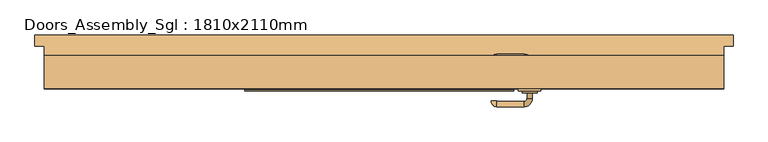
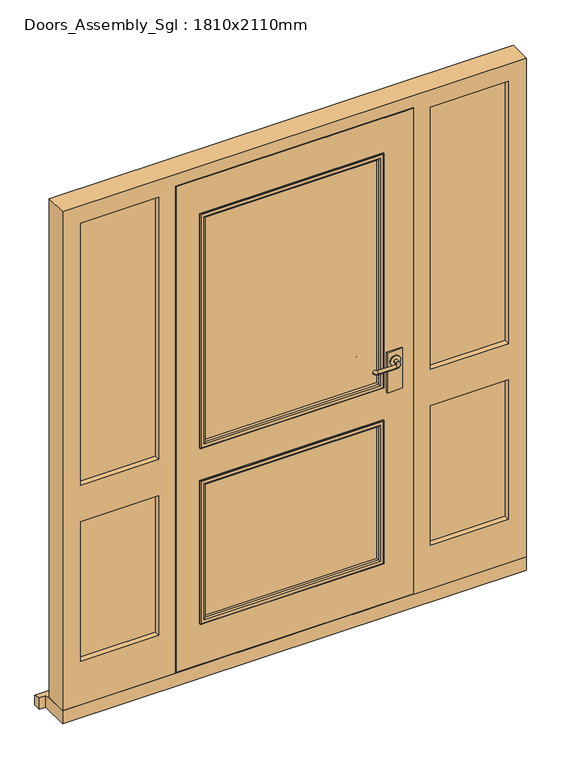
"""IFC4 building model written with IfcOpenShell, lengths in millimetres: door geometry, Doors_Assembly_Sgl : 1810x2110mm."""

from ifc_helpers import new_model, si_unit, point, frame, frame_2d, origin, place, context, project, spatial, polyline, circle_curve, ellipse_curve, trimmed, segment, composite_curve, outline, extrude, faceted_brep, source, transform, mapped, element, save
from ifc_brep_helpers import plane_surface, cylinder_surface, revolved_surface, advanced_brep


def doors_assembly_sgl_1810x2110mm_9edc52a6(model_context):
    return source(origin(), model_context, "Body", "SolidModel", [
        extrude(outline(composite_curve([segment(trimmed(circle_curve(frame_2d((1050.0, 680.0)), 20.0), [point((1050.0, 700.0))], [point((1050.0, 660.0))], False, "CARTESIAN"), True, "CONTINUOUS"), segment(trimmed(circle_curve(frame_2d((1050.0, 680.0)), 20.0), [point((1050.0, 660.0))], [point((1050.0, 700.0))], False, "CARTESIAN"), True, "CONTINUOUS")], self_intersect=False)), frame((0.0, 41.6570105, 0.0), z_axis=(0.0, 1.0, 0.0), x_axis=(0.0, 0.0, 1.0)), (0.0, 0.0, 1.0), 4.5929895),
        advanced_brep(
        [(673.0, 41.6570105, 1050.0), (687.0, 41.6570105, 1050.0), (673.0, 26.25, 1050.0), (687.0, 26.25, 1050.0), (665.0, 4.25, 1050.0), (665.0, 18.25, 1050.0), (593.0, 18.25, 1050.0), (593.0, 4.25, 1050.0), (592.0, 19.25, 1050.0), (578.0, 19.25, 1050.0)],
        [
            (0, 1, circle_curve(frame((680.0, 41.6570105, 1050.0), z_axis=(0.0, 1.0, 0.0), x_axis=(1.0, 0.0, 0.0)), 7.0)),
            (1, 0, circle_curve(frame((680.0, 41.6570105, 1050.0), z_axis=(0.0, 1.0, 0.0), x_axis=(1.0, 0.0, 0.0)), 7.0)),
            (0, 2),
            (2, 3, circle_curve(frame((680.0, 26.25, 1050.0), z_axis=(0.0, 1.0, 0.0), x_axis=(1.0, 0.0, 0.0)), 7.0)),
            (3, 1),
            (3, 2, circle_curve(frame((680.0, 26.25, 1050.0), z_axis=(0.0, 1.0, 0.0), x_axis=(1.0, 0.0, 0.0)), 7.0)),
            (4, 3, circle_curve(frame((665.0, 26.25, 1050.0), z_axis=(0.0, 0.0, 1.0), x_axis=(1.0, 0.0, 0.0)), 22.0)),
            (2, 5, circle_curve(frame((665.0, 26.25, 1050.0), z_axis=(0.0, 0.0, -1.0), x_axis=(1.0, 0.0, 0.0)), 8.0)),
            (5, 4, circle_curve(frame((665.0, 11.25, 1050.0), z_axis=(1.0, 0.0, 0.0), x_axis=(0.0, -1.0, 0.0)), 7.0)),
            (4, 5, circle_curve(frame((665.0, 11.25, 1050.0), z_axis=(1.0, 0.0, 0.0), x_axis=(0.0, -1.0, 0.0)), 7.0)),
            (5, 6),
            (6, 7, circle_curve(frame((593.0, 11.25, 1050.0), z_axis=(1.0, 0.0, 0.0), x_axis=(0.0, -1.0, 0.0)), 7.0)),
            (7, 4),
            (7, 6, circle_curve(frame((593.0, 11.25, 1050.0), z_axis=(1.0, 0.0, 0.0), x_axis=(0.0, -1.0, 0.0)), 7.0)),
            (8, 9, circle_curve(frame((585.0, 19.25, 1050.0), z_axis=(0.0, 1.0, 0.0), x_axis=(-1.0, 0.0, 0.0)), 7.0)),
            (9, 8, circle_curve(frame((585.0, 19.25, 1050.0), z_axis=(0.0, 1.0, 0.0), x_axis=(-1.0, 0.0, 0.0)), 7.0)),
            (9, 7, circle_curve(frame((593.0, 19.25, 1050.0), z_axis=(0.0, 0.0, 1.0), x_axis=(0.0, -1.0, 0.0)), 15.0)),
            (6, 8, circle_curve(frame((593.0, 19.25, 1050.0), z_axis=(0.0, 0.0, -1.0), x_axis=(0.0, -1.0, 0.0)), 1.0)),
        ],
        [
            plane_surface(frame((680.0, 41.6570105, 1050.0), z_axis=(0.0, 1.0, 0.0), x_axis=(0.0, 0.0, 1.0))),
            cylinder_surface(frame((680.0, 41.6570105, 1050.0), z_axis=(0.0, 1.0, 0.0), x_axis=(1.0, 0.0, 0.0)), 7.0),
            revolved_surface(trimmed(ellipse_curve(frame((680.0, 26.25, 1050.0), z_axis=(0.0, 1.0, 0.0), x_axis=(1.0, 0.0, 0.0)), 7.0, 7.0), [point((673.0, 26.25, 1050.0))], [point((687.0, 26.25, 1050.0))], True, "CARTESIAN"), (665.0, 26.25, 1050.0), (0.0, 0.0, -1.0)),
            revolved_surface(trimmed(ellipse_curve(frame((680.0, 26.25, 1050.0), z_axis=(0.0, 1.0, 0.0), x_axis=(1.0, 0.0, 0.0)), 7.0, 7.0), [point((687.0, 26.25, 1050.0))], [point((673.0, 26.25, 1050.0))], True, "CARTESIAN"), (665.0, 26.25, 1050.0), (0.0, 0.0, -1.0)),
            cylinder_surface(frame((665.0, 11.25, 1050.0), z_axis=(1.0, 0.0, 0.0), x_axis=(0.0, -1.0, 0.0)), 7.0),
            plane_surface(frame((585.0, 19.25, 1050.0), z_axis=(0.0, 1.0, 0.0), x_axis=(0.0, 0.0, 1.0))),
            revolved_surface(trimmed(ellipse_curve(frame((593.0, 11.25, 1050.0), z_axis=(1.0, 0.0, 0.0), x_axis=(0.0, -1.0, 0.0)), 7.0, 7.0), [point((593.0, 18.25, 1050.0))], [point((593.0, 4.25, 1050.0))], True, "CARTESIAN"), (593.0, 19.25, 1050.0), (0.0, 0.0, -1.0)),
            revolved_surface(trimmed(ellipse_curve(frame((593.0, 11.25, 1050.0), z_axis=(1.0, 0.0, 0.0), x_axis=(0.0, -1.0, 0.0)), 7.0, 7.0), [point((593.0, 4.25, 1050.0))], [point((593.0, 18.25, 1050.0))], True, "CARTESIAN"), (593.0, 19.25, 1050.0), (0.0, 0.0, -1.0)),
        ],
        [
            (0, [[1, 2]]),
            (1, [[-1, 3, 4, 5]]),
            (1, [[-2, -5, 6, -3]]),
            (2, [[7, -4, 8, 9]]),
            (3, [[-8, -6, -7, 10]]),
            (4, [[-9, 11, 12, 13]]),
            (4, [[-10, -13, 14, -11]]),
            (5, [[15, 16]]),
            (6, [[17, -12, 18, -16]]),
            (7, [[-18, -14, -17, -15]]),
        ],
    ),
        extrude(outline(polyline([(650.0, 52.25), (710.0, 52.25), (710.0, 46.25), (650.0, 46.25), (650.0, 52.25)])), frame((0.0, 0.0, 925.0), z_axis=(0.0, 0.0, 1.0), x_axis=(1.0, 0.0, 0.0)), (0.0, 0.0, 1.0), 165.0),
        extrude(outline(composite_curve([segment(trimmed(circle_curve(frame_2d((1050.0, 680.0)), 20.0), [point((1050.0, 700.0))], [point((1050.0, 660.0))], False, "CARTESIAN"), True, "CONTINUOUS"), segment(trimmed(circle_curve(frame_2d((1050.0, 680.0)), 20.0), [point((1050.0, 660.0))], [point((1050.0, 700.0))], False, "CARTESIAN"), True, "CONTINUOUS")], self_intersect=False)), frame((0.0, 102.25, 0.0), z_axis=(0.0, 1.0, 0.0), x_axis=(0.0, 0.0, 1.0)), (0.0, 0.0, 1.0), 4.5929895),
        advanced_brep(
        [(673.0, 106.8429895, 1050.0), (687.0, 106.8429895, 1050.0), (687.0, 122.25, 1050.0), (673.0, 122.25, 1050.0), (665.0, 144.25, 1050.0), (665.0, 130.25, 1050.0), (593.0, 144.25, 1050.0), (593.0, 130.25, 1050.0), (592.0, 129.25, 1050.0), (578.0, 129.25, 1050.0)],
        [
            (0, 1, circle_curve(frame((680.0, 106.8429895, 1050.0), z_axis=(0.0, -1.0, 0.0), x_axis=(1.0, 0.0, 0.0)), 7.0)),
            (1, 0, circle_curve(frame((680.0, 106.8429895, 1050.0), z_axis=(0.0, -1.0, 0.0), x_axis=(1.0, 0.0, 0.0)), 7.0)),
            (1, 2),
            (2, 3, circle_curve(frame((680.0, 122.25, 1050.0), z_axis=(0.0, -1.0, 0.0), x_axis=(1.0, 0.0, 0.0)), 7.0)),
            (3, 0),
            (3, 2, circle_curve(frame((680.0, 122.25, 1050.0), z_axis=(0.0, -1.0, 0.0), x_axis=(1.0, 0.0, 0.0)), 7.0)),
            (4, 5, circle_curve(frame((665.0, 137.25, 1050.0), z_axis=(1.0, 0.0, 0.0), x_axis=(0.0, 1.0, 0.0)), 7.0)),
            (5, 3, circle_curve(frame((665.0, 122.25, 1050.0), z_axis=(0.0, 0.0, -1.0), x_axis=(1.0, 0.0, 0.0)), 8.0)),
            (2, 4, circle_curve(frame((665.0, 122.25, 1050.0), z_axis=(0.0, 0.0, 1.0), x_axis=(1.0, 0.0, 0.0)), 22.0)),
            (5, 4, circle_curve(frame((665.0, 137.25, 1050.0), z_axis=(1.0, 0.0, 0.0), x_axis=(0.0, 1.0, 0.0)), 7.0)),
            (4, 6),
            (6, 7, circle_curve(frame((593.0, 137.25, 1050.0), z_axis=(1.0, 0.0, 0.0), x_axis=(0.0, 1.0, 0.0)), 7.0)),
            (7, 5),
            (7, 6, circle_curve(frame((593.0, 137.25, 1050.0), z_axis=(1.0, 0.0, 0.0), x_axis=(0.0, 1.0, 0.0)), 7.0)),
            (8, 9, circle_curve(frame((585.0, 129.25, 1050.0), z_axis=(0.0, -1.0, 0.0), x_axis=(-1.0, 0.0, 0.0)), 7.0)),
            (9, 8, circle_curve(frame((585.0, 129.25, 1050.0), z_axis=(0.0, -1.0, 0.0), x_axis=(-1.0, 0.0, 0.0)), 7.0)),
            (8, 7, circle_curve(frame((593.0, 129.25, 1050.0), z_axis=(0.0, 0.0, -1.0), x_axis=(0.0, 1.0, 0.0)), 1.0)),
            (6, 9, circle_curve(frame((593.0, 129.25, 1050.0), z_axis=(0.0, 0.0, 1.0), x_axis=(0.0, 1.0, 0.0)), 15.0)),
        ],
        [
            plane_surface(frame((680.0, 106.8429895, 1050.0), z_axis=(0.0, -1.0, 0.0), x_axis=(0.0, 0.0, 1.0))),
            cylinder_surface(frame((680.0, 106.8429895, 1050.0), z_axis=(0.0, -1.0, 0.0), x_axis=(1.0, 0.0, 0.0)), 7.0),
            revolved_surface(trimmed(ellipse_curve(frame((680.0, 122.25, 1050.0), z_axis=(0.0, 1.0, 0.0), x_axis=(1.0, 0.0, 0.0)), 7.0, 7.0), [point((673.0, 122.25, 1050.0))], [point((687.0, 122.25, 1050.0))], True, "CARTESIAN"), (665.0, 122.25, 1050.0), (0.0, 0.0, -1.0)),
            revolved_surface(trimmed(ellipse_curve(frame((680.0, 122.25, 1050.0), z_axis=(0.0, 1.0, 0.0), x_axis=(1.0, 0.0, 0.0)), 7.0, 7.0), [point((687.0, 122.25, 1050.0))], [point((673.0, 122.25, 1050.0))], True, "CARTESIAN"), (665.0, 122.25, 1050.0), (0.0, 0.0, -1.0)),
            cylinder_surface(frame((665.0, 137.25, 1050.0), z_axis=(1.0, 0.0, 0.0), x_axis=(0.0, 1.0, 0.0)), 7.0),
            plane_surface(frame((585.0, 129.25, 1050.0), z_axis=(0.0, -1.0, 0.0), x_axis=(0.0, 0.0, 1.0))),
            revolved_surface(trimmed(ellipse_curve(frame((593.0, 137.25, 1050.0), z_axis=(-1.0, 0.0, 0.0), x_axis=(0.0, 1.0, 0.0)), 7.0, 7.0), [point((593.0, 130.25, 1050.0))], [point((593.0, 144.25, 1050.0))], True, "CARTESIAN"), (593.0, 129.25, 1050.0), (0.0, 0.0, -1.0)),
            revolved_surface(trimmed(ellipse_curve(frame((593.0, 137.25, 1050.0), z_axis=(-1.0, 0.0, 0.0), x_axis=(0.0, 1.0, 0.0)), 7.0, 7.0), [point((593.0, 144.25, 1050.0))], [point((593.0, 130.25, 1050.0))], True, "CARTESIAN"), (593.0, 129.25, 1050.0), (0.0, 0.0, -1.0)),
        ],
        [
            (0, [[1, 2]]),
            (1, [[3, 4, 5, -2]]),
            (1, [[-5, 6, -3, -1]]),
            (2, [[7, 8, -4, 9]]),
            (3, [[10, -9, -6, -8]]),
            (4, [[11, 12, 13, -7]]),
            (4, [[-13, 14, -11, -10]]),
            (5, [[15, 16]]),
            (6, [[-15, 17, -12, 18]]),
            (7, [[-16, -18, -14, -17]]),
        ],
    ),
        extrude(outline(polyline([(650.0, 96.25), (650.0, 102.25), (710.0, 102.25), (710.0, 96.25), (650.0, 96.25)])), frame((0.0, 0.0, 925.0), z_axis=(0.0, 0.0, 1.0), x_axis=(1.0, 0.0, 0.0)), (0.0, 0.0, 1.0), 165.0),
        extrude(outline(polyline([(1148.5, 75.25), (800.0, 75.25), (800.0, 99.25), (1148.5, 99.25), (1148.5, 75.25)])), frame((0.0, 0.0, 218.5), z_axis=(0.0, 0.0, 1.0), x_axis=(1.0, 0.0, 0.0)), (0.0, 0.0, 1.0), 605.0),
        extrude(outline(polyline([(1148.5, 75.25), (800.0, 75.25), (800.0, 99.25), (1148.5, 99.25), (1148.5, 75.25)])), frame((0.0, 0.0, 943.5), z_axis=(0.0, 0.0, 1.0), x_axis=(1.0, 0.0, 0.0)), (0.0, 0.0, 1.0), 1118.0),
        extrude(outline(polyline([(-216.0, 75.25), (-564.5, 75.25), (-564.5, 99.25), (-216.0, 99.25), (-216.0, 75.25)])), frame((0.0, 0.0, 943.5), z_axis=(0.0, 0.0, 1.0), x_axis=(1.0, 0.0, 0.0)), (0.0, 0.0, 1.0), 1118.0),
        extrude(outline(polyline([(-216.0, 75.25), (-564.5, 75.25), (-564.5, 99.25), (-216.0, 99.25), (-216.0, 75.25)])), frame((0.0, 0.0, 218.5), z_axis=(0.0, 0.0, 1.0), x_axis=(1.0, 0.0, 0.0)), (0.0, 0.0, 1.0), 605.0),
        faceted_brep([(1197.0, 141.25, 54.5), (1197.0, 52.25, 54.5), (758.0, 52.25, 54.5), (758.0, 99.25, 54.5), (736.0, 99.25, 54.5), (736.0, 141.25, 54.5), (1197.0, 141.25, 2110.0), (1197.0, 52.25, 2110.0), (-613.0, 52.25, 2110.0), (-613.0, 52.25, 54.5), (-174.0, 52.25, 54.5), (-174.0, 52.25, 2061.5), (758.0, 52.25, 2061.5), (1126.5, 52.25, 958.5), (822.0, 52.25, 958.5), (822.0, 52.25, 2039.5), (1126.5, 52.25, 2039.5), (822.0, 52.25, 808.5), (1126.5, 52.25, 808.5), (1126.5, 52.25, 233.5), (822.0, 52.25, 233.5), (-238.0, 52.25, 808.5), (-238.0, 52.25, 233.5), (-542.5, 52.25, 233.5), (-542.5, 52.25, 808.5), (-542.5, 52.25, 2039.5), (-238.0, 52.25, 2039.5), (-238.0, 52.25, 958.5), (-542.5, 52.25, 958.5), (758.0, 99.25, 2061.5), (-174.0, 99.25, 54.5), (-152.0, 99.25, 54.5), (-152.0, 99.25, 2039.5), (736.0, 99.25, 2039.5), (-174.0, 99.25, 2061.5), (1148.5, 99.25, 218.5), (1148.5, 99.25, 823.5), (800.0, 99.25, 823.5), (800.0, 99.25, 218.5), (1126.5, 99.25, 808.5), (1126.5, 99.25, 233.5), (822.0, 99.25, 233.5), (822.0, 99.25, 808.5), (-564.5, 99.25, 823.5), (-564.5, 99.25, 218.5), (-216.0, 99.25, 218.5), (-216.0, 99.25, 823.5), (-238.0, 99.25, 808.5), (-238.0, 99.25, 233.5), (-542.5, 99.25, 233.5), (-542.5, 99.25, 808.5), (-216.0, 99.25, 2061.5), (-564.5, 99.25, 2061.5), (-564.5, 99.25, 943.5), (-216.0, 99.25, 943.5), (-542.5, 99.25, 2039.5), (-238.0, 99.25, 2039.5), (-238.0, 99.25, 958.5), (-542.5, 99.25, 958.5), (1148.5, 99.25, 2061.5), (800.0, 99.25, 2061.5), (800.0, 99.25, 943.5), (1148.5, 99.25, 943.5), (822.0, 99.25, 2039.5), (1126.5, 99.25, 2039.5), (1126.5, 99.25, 958.5), (822.0, 99.25, 958.5), (736.0, 141.25, 2039.5), (-613.0, 141.25, 54.5), (-613.0, 141.25, 2110.0), (-152.0, 141.25, 2039.5), (-152.0, 141.25, 54.5), (-238.0, 141.25, 2039.5), (-542.5, 141.25, 2039.5), (-542.5, 141.25, 233.5), (-238.0, 141.25, 233.5), (1126.5, 141.25, 2039.5), (822.0, 141.25, 2039.5), (822.0, 141.25, 233.5), (1126.5, 141.25, 233.5), (-542.5, 122.25, 958.5), (-542.5, 122.25, 808.5), (-238.0, 122.25, 808.5), (-238.0, 122.25, 958.5), (822.0, 122.25, 958.5), (822.0, 122.25, 808.5), (1126.5, 122.25, 808.5), (1126.5, 122.25, 958.5), (1126.5, 75.25, 958.5), (822.0, 75.25, 958.5), (822.0, 75.25, 233.5), (822.0, 75.25, 808.5), (822.0, 75.25, 2039.5), (1126.5, 75.25, 808.5), (1126.5, 75.25, 233.5), (1126.5, 75.25, 2039.5), (-238.0, 75.25, 808.5), (-238.0, 75.25, 233.5), (-238.0, 75.25, 2039.5), (-238.0, 75.25, 958.5), (-542.5, 75.25, 233.5), (-542.5, 75.25, 808.5), (-542.5, 75.25, 2039.5), (-542.5, 75.25, 958.5), (1148.5, 75.25, 218.5), (1148.5, 75.25, 823.5), (1148.5, 75.25, 943.5), (1148.5, 75.25, 2061.5), (800.0, 75.25, 218.5), (800.0, 75.25, 823.5), (800.0, 75.25, 2061.5), (800.0, 75.25, 943.5), (-564.5, 75.25, 218.5), (-564.5, 75.25, 823.5), (-564.5, 75.25, 943.5), (-564.5, 75.25, 2061.5), (-216.0, 75.25, 943.5), (-216.0, 75.25, 2061.5), (-216.0, 75.25, 218.5), (-216.0, 75.25, 823.5)], [[[0, 1, 2, 3, 4, 5]], [[1, 0, 6, 7]], [[1, 7, 8, 9, 10, 11, 12, 2], [13, 14, 15, 16], [17, 18, 19, 20], [21, 22, 23, 24], [25, 26, 27, 28]], [[3, 2, 12, 29]], [[30, 31, 32, 33, 4, 3, 29, 34]], [[35, 36, 37, 38], [39, 40, 41, 42]], [[43, 44, 45, 46], [47, 48, 49, 50]], [[51, 52, 53, 54], [55, 56, 57, 58]], [[59, 60, 61, 62], [63, 64, 65, 66]], [[5, 4, 33, 67]], [[68, 69, 6, 0, 5, 67, 70, 71], [72, 73, 74, 75], [76, 77, 78, 79]], [[69, 68, 9, 8]], [[31, 71, 70, 32]], [[9, 68, 71, 31, 30, 10]], [[73, 55, 58, 80, 81, 50, 49, 74]], [[49, 48, 75, 74]], [[56, 72, 75, 48, 47, 82, 83, 57]], [[77, 63, 66, 84, 85, 42, 41, 78]], [[79, 78, 41, 40]], [[64, 76, 79, 40, 39, 86, 87, 65]], [[14, 13, 88, 89]], [[17, 20, 90, 91]], [[92, 15, 14, 89]], [[19, 18, 93, 94]], [[16, 95, 88, 13]], [[18, 17, 91, 93]], [[20, 19, 94, 90]], [[22, 21, 96, 97]], [[26, 98, 99, 27]], [[23, 22, 97, 100]], [[24, 23, 100, 101]], [[102, 25, 28, 103]], [[21, 24, 101, 96]], [[28, 27, 99, 103]], [[10, 30, 34, 11]], [[104, 105, 36, 35]], [[106, 107, 59, 62]], [[104, 108, 109, 105], [94, 93, 91, 90]], [[110, 107, 106, 111], [95, 92, 89, 88]], [[36, 105, 109, 37]], [[108, 104, 35, 38]], [[111, 106, 62, 61]], [[58, 57, 83, 80]], [[112, 44, 43, 113]], [[114, 53, 52, 115]], [[53, 114, 116, 54]], [[54, 116, 117, 51]], [[45, 118, 119, 46]], [[66, 65, 87, 84]], [[110, 111, 61, 60]], [[109, 108, 38, 37]], [[39, 42, 85, 86]], [[47, 50, 81, 82]], [[112, 118, 45, 44]], [[113, 43, 46, 119]], [[84, 87, 86, 85]], [[118, 112, 113, 119], [100, 97, 96, 101]], [[115, 117, 116, 114], [98, 102, 103, 99]], [[80, 83, 82, 81]], [[6, 69, 8, 7]], [[52, 51, 117, 115]], [[60, 59, 107, 110]], [[11, 34, 29, 12]], [[76, 64, 63, 77]], [[55, 73, 72, 56]], [[32, 70, 67, 33]], [[102, 98, 26, 25]], [[16, 15, 92, 95]]]),
        extrude(outline(polyline([(-71.0, 86.25), (630.0, 86.25), (630.0, 62.25), (-71.0, 62.25), (-71.0, 86.25)])), frame((0.0, 0.0, 958.5), z_axis=(0.0, 0.0, 1.0), x_axis=(1.0, 0.0, 0.0)), (0.0, 0.0, 1.0), 950.0),
        extrude(outline(polyline([(-71.0, 86.25), (630.0, 86.25), (630.0, 62.25), (-71.0, 62.25), (-71.0, 86.25)])), frame((0.0, 0.0, 233.5), z_axis=(0.0, 0.0, 1.0), x_axis=(1.0, 0.0, 0.0)), (0.0, 0.0, 1.0), 575.0),
        faceted_brep([(1222.0, 196.25, 0.0), (1222.0, 196.25, 38.5947221), (1222.0, 166.25, 47.2703282), (1222.0, 166.25, 0.0), (-638.0, 196.25, 38.5947221), (-638.0, 196.25, 0.0), (-638.0, 166.25, 0.0), (-638.0, 166.25, 47.2703282), (1197.0, 166.25, 0.0), (1197.0, 52.25, 0.0), (-613.0, 52.25, 0.0), (-613.0, 166.25, 0.0), (-613.0, 166.25, 47.2703282), (-613.0, 141.25, 54.5), (1197.0, 141.25, 54.5), (1197.0, 166.25, 47.2703282), (-613.0, 52.25, 54.5), (1197.0, 52.25, 54.5)], [[[0, 1, 2, 3]], [[4, 5, 6, 7]], [[5, 0, 3, 8, 9, 10, 11, 6]], [[1, 0, 5, 4]], [[1, 4, 7, 12, 13, 14, 15, 2]], [[13, 16, 17, 14]], [[16, 10, 9, 17]], [[12, 11, 10, 16, 13]], [[11, 12, 7, 6]], [[8, 15, 14, 17, 9]], [[15, 8, 3, 2]]]),
        extrude(outline(polyline([(58.5, -171.0), (58.5, 755.0), (2058.5, 755.0), (2058.5, -171.0), (58.5, -171.0)]), holes=[polyline([(1908.5, 630.0), (958.5, 630.0), (958.5, -71.0), (1908.5, -71.0), (1908.5, 630.0)]), polyline([(808.5, -71.0), (808.5, 630.0), (233.5, 630.0), (233.5, -71.0), (808.5, -71.0)])]), frame((0.0, 52.25, 0.0), z_axis=(0.0, 1.0, 0.0), x_axis=(0.0, 0.0, 1.0)), (0.0, 0.0, 1.0), 44.0),
        advanced_brep(
        [(630.0, 62.25, 808.5), (630.0, 52.25, 808.5), (630.0, 52.25, 233.5), (630.0, 62.25, 233.5), (618.0, 51.25, 796.5), (618.0, 62.25, 796.5), (618.0, 62.25, 245.5), (618.0, 51.25, 245.5), (623.0, 46.25, 801.5), (623.0, 46.25, 240.5), (638.0, 48.25, 816.5), (636.0, 46.25, 814.5), (636.0, 46.25, 227.5), (638.0, 48.25, 225.5), (638.0, 52.25, 816.5), (638.0, 52.25, 225.5), (-71.0, 52.25, 233.5), (-71.0, 62.25, 233.5), (-59.0, 62.25, 245.5), (-59.0, 51.25, 245.5), (-64.0, 46.25, 240.5), (-77.0, 46.25, 227.5), (-79.0, 48.25, 225.5), (-79.0, 52.25, 225.5), (-71.0, 52.25, 808.5), (-71.0, 62.25, 808.5), (-59.0, 62.25, 796.5), (-59.0, 51.25, 796.5), (-64.0, 46.25, 801.5), (-77.0, 46.25, 814.5), (-79.0, 48.25, 816.5), (-79.0, 52.25, 816.5)],
        [
            (0, 1),
            (1, 2),
            (2, 3),
            (3, 0),
            (4, 5),
            (5, 6),
            (6, 7),
            (7, 4),
            (8, 4, ellipse_curve(frame((623.0, 51.25, 801.5), z_axis=(0.707106781186552, 0.0, -0.707106781186543), x_axis=(0.7071067811865429, 0.0, 0.707106781186552)), 7.0710678, 5.0)),
            (7, 9, ellipse_curve(frame((623.0, 51.25, 240.5), z_axis=(0.7071067811865429, 0.0, 0.707106781186552), x_axis=(-0.7071067811865519, 0.0, 0.7071067811865431)), 7.0710678, 5.0)),
            (9, 8),
            (10, 11, ellipse_curve(frame((636.0, 48.25, 814.5), z_axis=(0.707106781186552, 0.0, -0.707106781186543), x_axis=(0.7071067811865429, 0.0, 0.707106781186552)), 2.8284271, 2.0)),
            (11, 12),
            (12, 13, ellipse_curve(frame((636.0, 48.25, 227.5), z_axis=(0.7071067811865429, 0.0, 0.707106781186552), x_axis=(-0.7071067811865519, 0.0, 0.7071067811865431)), 2.8284271, 2.0)),
            (13, 10),
            (14, 10),
            (13, 15),
            (15, 14),
            (2, 16),
            (16, 17),
            (17, 3),
            (6, 18),
            (18, 19),
            (19, 7),
            (19, 20, ellipse_curve(frame((-64.0, 51.25, 240.5), z_axis=(0.707106781186552, 0.0, -0.7071067811865431), x_axis=(0.7071067811865429, 0.0, 0.707106781186552)), 7.0710678, 5.0)),
            (20, 9),
            (12, 21),
            (21, 22, ellipse_curve(frame((-77.0, 48.25, 227.5), z_axis=(0.707106781186552, 0.0, -0.7071067811865431), x_axis=(0.7071067811865429, 0.0, 0.707106781186552)), 2.8284271, 2.0)),
            (22, 13),
            (22, 23),
            (23, 15),
            (16, 24),
            (24, 25),
            (25, 17),
            (18, 26),
            (26, 27),
            (27, 19),
            (27, 28, ellipse_curve(frame((-64.0, 51.25, 801.5), z_axis=(-0.707106781186543, 0.0, -0.7071067811865519), x_axis=(0.7071067811865518, 0.0, -0.7071067811865431)), 7.0710678, 5.0)),
            (28, 20),
            (21, 29),
            (29, 30, ellipse_curve(frame((-77.0, 48.25, 814.5), z_axis=(-0.707106781186543, 0.0, -0.7071067811865519), x_axis=(0.7071067811865518, 0.0, -0.7071067811865431)), 2.8284271, 2.0)),
            (30, 22),
            (30, 31),
            (31, 23),
            (31, 14),
            (1, 24),
            (0, 25),
            (5, 26),
            (4, 27),
            (8, 28),
            (11, 29),
            (10, 30),
        ],
        [
            plane_surface(frame((630.0, 52.25, 808.5), z_axis=(1.0, 0.0, 0.0), x_axis=(0.0, 0.0, -1.0))),
            plane_surface(frame((618.0, 62.25, 796.5), z_axis=(-1.0, 0.0, 0.0), x_axis=(0.0, 0.0, -1.0))),
            cylinder_surface(frame((623.0, 51.25, 808.5), z_axis=(0.0, 0.0, 1.0), x_axis=(1.0, 0.0, 0.0)), 5.0),
            cylinder_surface(frame((636.0, 48.25, 808.5), z_axis=(0.0, 0.0, 1.0), x_axis=(1.0, 0.0, 0.0)), 2.0),
            plane_surface(frame((638.0, 48.25, 816.5), z_axis=(1.0, 0.0, 0.0), x_axis=(0.0, 0.0, -1.0))),
            plane_surface(frame((630.0, 52.25, 233.5), z_axis=(0.0, 0.0, -1.0), x_axis=(-1.0, 0.0, 0.0))),
            plane_surface(frame((618.0, 62.25, 245.5), z_axis=(0.0, 0.0, 1.0), x_axis=(-1.0, 0.0, 0.0))),
            cylinder_surface(frame((630.0, 51.25, 240.5), z_axis=(1.0, 0.0, 0.0), x_axis=(0.0, 0.0, -1.0)), 5.0),
            cylinder_surface(frame((630.0, 48.25, 227.5), z_axis=(1.0, 0.0, 0.0), x_axis=(0.0, 0.0, -1.0)), 2.0),
            plane_surface(frame((638.0, 48.25, 225.5), z_axis=(0.0, 0.0, -1.0), x_axis=(-1.0, 0.0, 0.0))),
            plane_surface(frame((-71.0, 52.25, 233.5), z_axis=(-1.0, 0.0, 0.0), x_axis=(0.0, 0.0, 1.0))),
            plane_surface(frame((-59.0, 62.25, 245.5), z_axis=(1.0, 0.0, 0.0), x_axis=(0.0, 0.0, 1.0))),
            cylinder_surface(frame((-64.0, 51.25, 233.5), z_axis=(0.0, 0.0, -1.0), x_axis=(-1.0, 0.0, 0.0)), 5.0),
            cylinder_surface(frame((-77.0, 48.25, 233.5), z_axis=(0.0, 0.0, -1.0), x_axis=(-1.0, 0.0, 0.0)), 2.0),
            plane_surface(frame((-79.0, 48.25, 225.5), z_axis=(-1.0, 0.0, 0.0), x_axis=(0.0, 0.0, 1.0))),
            plane_surface(frame((-79.0, 52.25, 816.5), z_axis=(0.0, 1.0, 0.0), x_axis=(1.0, 0.0, 0.0))),
            plane_surface(frame((-71.0, 52.25, 808.5), z_axis=(0.0, 0.0, 1.0), x_axis=(1.0, 0.0, 0.0))),
            plane_surface(frame((-71.0, 62.25, 808.5), z_axis=(0.0, 1.0, 0.0), x_axis=(1.0, 0.0, 0.0))),
            plane_surface(frame((-59.0, 62.25, 796.5), z_axis=(0.0, 0.0, -1.0), x_axis=(1.0, 0.0, 0.0))),
            cylinder_surface(frame((-71.0, 51.25, 801.5), z_axis=(-1.0, 0.0, 0.0), x_axis=(0.0, 0.0, 1.0)), 5.0),
            plane_surface(frame((-64.0, 46.25, 801.5), z_axis=(0.0, -1.0, 0.0), x_axis=(1.0, 0.0, 0.0))),
            cylinder_surface(frame((-71.0, 48.25, 814.5), z_axis=(-1.0, 0.0, 0.0), x_axis=(0.0, 0.0, 1.0)), 2.0),
            plane_surface(frame((-79.0, 48.25, 816.5), z_axis=(0.0, 0.0, 1.0), x_axis=(1.0, 0.0, 0.0))),
        ],
        [
            (0, [[1, 2, 3, 4]]),
            (1, [[5, 6, 7, 8]]),
            (2, [[9, -8, 10, 11]]),
            (3, [[12, 13, 14, 15]]),
            (4, [[16, -15, 17, 18]]),
            (5, [[-3, 19, 20, 21]]),
            (6, [[-7, 22, 23, 24]]),
            (7, [[-10, -24, 25, 26]]),
            (8, [[-14, 27, 28, 29]]),
            (9, [[-17, -29, 30, 31]]),
            (10, [[-20, 32, 33, 34]]),
            (11, [[-23, 35, 36, 37]]),
            (12, [[-25, -37, 38, 39]]),
            (13, [[-28, 40, 41, 42]]),
            (14, [[-30, -42, 43, 44]]),
            (15, [[-31, -44, 45, -18], [46, -32, -19, -2]]),
            (16, [[-33, -46, -1, 47]]),
            (17, [[-21, -34, -47, -4], [48, -35, -22, -6]]),
            (18, [[-36, -48, -5, 49]]),
            (19, [[-38, -49, -9, 50]]),
            (20, [[51, -40, -27, -13], [-26, -39, -50, -11]]),
            (21, [[-41, -51, -12, 52]]),
            (22, [[-43, -52, -16, -45]]),
        ],
    ),
        advanced_brep(
        [(-71.0, 86.25, 808.5), (-71.0, 96.25, 808.5), (-71.0, 96.25, 233.5), (-71.0, 86.25, 233.5), (-59.0, 97.25, 796.5), (-59.0, 86.25, 796.5), (-59.0, 86.25, 245.5), (-59.0, 97.25, 245.5), (-64.0, 102.25, 801.5), (-64.0, 102.25, 240.5), (-79.0, 100.25, 816.5), (-77.0, 102.25, 814.5), (-77.0, 102.25, 227.5), (-79.0, 100.25, 225.5), (-79.0, 96.25, 816.5), (-79.0, 96.25, 225.5), (630.0, 96.25, 233.5), (630.0, 86.25, 233.5), (618.0, 86.25, 245.5), (618.0, 97.25, 245.5), (623.0, 102.25, 240.5), (636.0, 102.25, 227.5), (638.0, 100.25, 225.5), (638.0, 96.25, 225.5), (630.0, 96.25, 808.5), (630.0, 86.25, 808.5), (618.0, 86.25, 796.5), (618.0, 97.25, 796.5), (623.0, 102.25, 801.5), (636.0, 102.25, 814.5), (638.0, 100.25, 816.5), (638.0, 96.25, 816.5)],
        [
            (0, 1),
            (1, 2),
            (2, 3),
            (3, 0),
            (4, 5),
            (5, 6),
            (6, 7),
            (7, 4),
            (8, 4, ellipse_curve(frame((-64.0, 97.25, 801.5), z_axis=(-0.7071067811865475, 0.0, -0.7071067811865475), x_axis=(-0.7071067811865474, 0.0, 0.7071067811865477)), 7.0710678, 5.0)),
            (7, 9, ellipse_curve(frame((-64.0, 97.25, 240.5), z_axis=(-0.7071067811865475, 0.0, 0.7071067811865475), x_axis=(0.7071067811865474, 0.0, 0.7071067811865476)), 7.0710678, 5.0)),
            (9, 8),
            (10, 11, ellipse_curve(frame((-77.0, 100.25, 814.5), z_axis=(-0.7071067811865475, 0.0, -0.7071067811865475), x_axis=(-0.7071067811865474, 0.0, 0.7071067811865477)), 2.8284271, 2.0)),
            (11, 12),
            (12, 13, ellipse_curve(frame((-77.0, 100.25, 227.5), z_axis=(-0.7071067811865475, 0.0, 0.7071067811865475), x_axis=(0.7071067811865474, 0.0, 0.7071067811865476)), 2.8284271, 2.0)),
            (13, 10),
            (14, 10),
            (13, 15),
            (15, 14),
            (2, 16),
            (16, 17),
            (17, 3),
            (6, 18),
            (18, 19),
            (19, 7),
            (19, 20, ellipse_curve(frame((623.0, 97.25, 240.5), z_axis=(-0.7071067811865475, 0.0, -0.7071067811865475), x_axis=(-0.7071067811865476, 0.0, 0.7071067811865474)), 7.0710678, 5.0)),
            (20, 9),
            (12, 21),
            (21, 22, ellipse_curve(frame((636.0, 100.25, 227.5), z_axis=(-0.7071067811865475, 0.0, -0.7071067811865475), x_axis=(-0.7071067811865476, 0.0, 0.7071067811865474)), 2.8284271, 2.0)),
            (22, 13),
            (22, 23),
            (23, 15),
            (16, 24),
            (24, 25),
            (25, 17),
            (18, 26),
            (26, 27),
            (27, 19),
            (27, 28, ellipse_curve(frame((623.0, 97.25, 801.5), z_axis=(0.7071067811865475, 0.0, -0.7071067811865475), x_axis=(-0.7071067811865474, 0.0, -0.7071067811865477)), 7.0710678, 5.0)),
            (28, 20),
            (21, 29),
            (29, 30, ellipse_curve(frame((636.0, 100.25, 814.5), z_axis=(0.7071067811865475, 0.0, -0.7071067811865475), x_axis=(-0.7071067811865474, 0.0, -0.7071067811865477)), 2.8284271, 2.0)),
            (30, 22),
            (30, 31),
            (31, 23),
            (31, 14),
            (1, 24),
            (0, 25),
            (5, 26),
            (4, 27),
            (8, 28),
            (11, 29),
            (10, 30),
        ],
        [
            plane_surface(frame((-71.0, 96.25, 808.5), z_axis=(-1.0, 0.0, 0.0), x_axis=(0.0, 0.0, -1.0))),
            plane_surface(frame((-59.0, 86.25, 796.5), z_axis=(1.0, 0.0, 0.0), x_axis=(0.0, 0.0, -1.0))),
            cylinder_surface(frame((-64.0, 97.25, 808.5), z_axis=(0.0, 0.0, 1.0), x_axis=(-1.0, 0.0, 0.0)), 5.0),
            cylinder_surface(frame((-77.0, 100.25, 808.5), z_axis=(0.0, 0.0, 1.0), x_axis=(-1.0, 0.0, 0.0)), 2.0),
            plane_surface(frame((-79.0, 100.25, 816.5), z_axis=(-1.0, 0.0, 0.0), x_axis=(0.0, 0.0, -1.0))),
            plane_surface(frame((-71.0, 96.25, 233.5), z_axis=(0.0, 0.0, -1.0), x_axis=(1.0, 0.0, 0.0))),
            plane_surface(frame((-59.0, 86.25, 245.5), z_axis=(0.0, 0.0, 1.0), x_axis=(1.0, 0.0, 0.0))),
            cylinder_surface(frame((-71.0, 97.25, 240.5), z_axis=(-1.0, 0.0, 0.0), x_axis=(0.0, 0.0, -1.0)), 5.0),
            cylinder_surface(frame((-71.0, 100.25, 227.5), z_axis=(-1.0, 0.0, 0.0), x_axis=(0.0, 0.0, -1.0)), 2.0),
            plane_surface(frame((-79.0, 100.25, 225.5), z_axis=(0.0, 0.0, -1.0), x_axis=(1.0, 0.0, 0.0))),
            plane_surface(frame((630.0, 96.25, 233.5), z_axis=(1.0, 0.0, 0.0), x_axis=(0.0, 0.0, 1.0))),
            plane_surface(frame((618.0, 86.25, 245.5), z_axis=(-1.0, 0.0, 0.0), x_axis=(0.0, 0.0, 1.0))),
            cylinder_surface(frame((623.0, 97.25, 233.5), z_axis=(0.0, 0.0, -1.0), x_axis=(1.0, 0.0, 0.0)), 5.0),
            cylinder_surface(frame((636.0, 100.25, 233.5), z_axis=(0.0, 0.0, -1.0), x_axis=(1.0, 0.0, 0.0)), 2.0),
            plane_surface(frame((638.0, 100.25, 225.5), z_axis=(1.0, 0.0, 0.0), x_axis=(0.0, 0.0, 1.0))),
            plane_surface(frame((638.0, 96.25, 816.5), z_axis=(0.0, -1.0, 0.0), x_axis=(-1.0, 0.0, 0.0))),
            plane_surface(frame((630.0, 96.25, 808.5), z_axis=(0.0, 0.0, 1.0), x_axis=(-1.0, 0.0, 0.0))),
            plane_surface(frame((630.0, 86.25, 808.5), z_axis=(0.0, -1.0, 0.0), x_axis=(-1.0, 0.0, 0.0))),
            plane_surface(frame((618.0, 86.25, 796.5), z_axis=(0.0, 0.0, -1.0), x_axis=(-1.0, 0.0, 0.0))),
            cylinder_surface(frame((630.0, 97.25, 801.5), z_axis=(1.0, 0.0, 0.0), x_axis=(0.0, 0.0, 1.0)), 5.0),
            plane_surface(frame((623.0, 102.25, 801.5), z_axis=(0.0, 1.0, 0.0), x_axis=(-1.0, 0.0, 0.0))),
            cylinder_surface(frame((630.0, 100.25, 814.5), z_axis=(1.0, 0.0, 0.0), x_axis=(0.0, 0.0, 1.0)), 2.0),
            plane_surface(frame((638.0, 100.25, 816.5), z_axis=(0.0, 0.0, 1.0), x_axis=(-1.0, 0.0, 0.0))),
        ],
        [
            (0, [[1, 2, 3, 4]]),
            (1, [[5, 6, 7, 8]]),
            (2, [[9, -8, 10, 11]]),
            (3, [[12, 13, 14, 15]]),
            (4, [[16, -15, 17, 18]]),
            (5, [[-3, 19, 20, 21]]),
            (6, [[-7, 22, 23, 24]]),
            (7, [[-10, -24, 25, 26]]),
            (8, [[-14, 27, 28, 29]]),
            (9, [[-17, -29, 30, 31]]),
            (10, [[-20, 32, 33, 34]]),
            (11, [[-23, 35, 36, 37]]),
            (12, [[-25, -37, 38, 39]]),
            (13, [[-28, 40, 41, 42]]),
            (14, [[-30, -42, 43, 44]]),
            (15, [[-31, -44, 45, -18], [46, -32, -19, -2]]),
            (16, [[-33, -46, -1, 47]]),
            (17, [[-21, -34, -47, -4], [48, -35, -22, -6]]),
            (18, [[-36, -48, -5, 49]]),
            (19, [[-38, -49, -9, 50]]),
            (20, [[51, -40, -27, -13], [-26, -39, -50, -11]]),
            (21, [[-41, -51, -12, 52]]),
            (22, [[-43, -52, -16, -45]]),
        ],
    ),
        advanced_brep(
        [(-79.0, 100.25, 950.5), (-79.0, 96.25, 950.5), (-79.0, 96.25, 1916.5), (-79.0, 100.25, 1916.5), (-77.0, 102.25, 952.5), (-77.0, 102.25, 1914.5), (-59.0, 97.25, 970.5), (-64.0, 102.25, 965.5), (-64.0, 102.25, 1901.5), (-59.0, 97.25, 1896.5), (-59.0, 86.25, 970.5), (-59.0, 86.25, 1896.5), (-71.0, 96.25, 958.5), (-71.0, 86.25, 958.5), (-71.0, 86.25, 1908.5), (-71.0, 96.25, 1908.5), (638.0, 96.25, 1916.5), (638.0, 100.25, 1916.5), (636.0, 102.25, 1914.5), (623.0, 102.25, 1901.5), (618.0, 97.25, 1896.5), (618.0, 86.25, 1896.5), (630.0, 86.25, 1908.5), (630.0, 96.25, 1908.5), (638.0, 96.25, 950.5), (638.0, 100.25, 950.5), (636.0, 102.25, 952.5), (623.0, 102.25, 965.5), (618.0, 97.25, 970.5), (618.0, 86.25, 970.5), (630.0, 86.25, 958.5), (630.0, 96.25, 958.5)],
        [
            (0, 1),
            (1, 2),
            (2, 3),
            (3, 0),
            (4, 0, ellipse_curve(frame((-77.0, 100.25, 952.5), z_axis=(-0.7071067811865474, 0.0, 0.7071067811865476), x_axis=(-0.7071067811865475, 0.0, -0.7071067811865475)), 2.8284271, 2.0)),
            (3, 5, ellipse_curve(frame((-77.0, 100.25, 1914.5), z_axis=(-0.7071067811865476, 0.0, -0.7071067811865474), x_axis=(0.7071067811865472, 0.0, -0.7071067811865478)), 2.8284271, 2.0)),
            (5, 4),
            (6, 7, ellipse_curve(frame((-64.0, 97.25, 965.5), z_axis=(-0.7071067811865474, 0.0, 0.7071067811865476), x_axis=(-0.7071067811865475, 0.0, -0.7071067811865475)), 7.0710678, 5.0)),
            (7, 8),
            (8, 9, ellipse_curve(frame((-64.0, 97.25, 1901.5), z_axis=(-0.7071067811865476, 0.0, -0.7071067811865474), x_axis=(0.7071067811865472, 0.0, -0.7071067811865478)), 7.0710678, 5.0)),
            (9, 6),
            (10, 6),
            (9, 11),
            (11, 10),
            (12, 13),
            (13, 14),
            (14, 15),
            (15, 12),
            (2, 16),
            (16, 17),
            (17, 3),
            (17, 18, ellipse_curve(frame((636.0, 100.25, 1914.5), z_axis=(-0.7071067811865474, 0.0, 0.7071067811865476), x_axis=(-0.7071067811865477, 0.0, -0.7071067811865472)), 2.8284271, 2.0)),
            (18, 5),
            (8, 19),
            (19, 20, ellipse_curve(frame((623.0, 97.25, 1901.5), z_axis=(-0.7071067811865474, 0.0, 0.7071067811865476), x_axis=(-0.7071067811865477, 0.0, -0.7071067811865472)), 7.0710678, 5.0)),
            (20, 9),
            (20, 21),
            (21, 11),
            (14, 22),
            (22, 23),
            (23, 15),
            (16, 24),
            (24, 25),
            (25, 17),
            (25, 26, ellipse_curve(frame((636.0, 100.25, 952.5), z_axis=(0.7071067811865476, 0.0, 0.7071067811865474), x_axis=(-0.7071067811865474, 0.0, 0.7071067811865477)), 2.8284271, 2.0)),
            (26, 18),
            (19, 27),
            (27, 28, ellipse_curve(frame((623.0, 97.25, 965.5), z_axis=(0.7071067811865476, 0.0, 0.7071067811865474), x_axis=(-0.7071067811865474, 0.0, 0.7071067811865477)), 7.0710678, 5.0)),
            (28, 20),
            (28, 29),
            (29, 21),
            (22, 30),
            (30, 31),
            (31, 23),
            (24, 1),
            (0, 25),
            (4, 26),
            (7, 27),
            (6, 28),
            (10, 29),
            (13, 30),
            (12, 31),
        ],
        [
            plane_surface(frame((-79.0, 96.25, 950.5), z_axis=(-1.0, 0.0, 0.0), x_axis=(0.0, 0.0, 1.0))),
            cylinder_surface(frame((-77.0, 100.25, 958.5), z_axis=(0.0, 0.0, -1.0), x_axis=(-1.0, 0.0, 0.0)), 2.0),
            cylinder_surface(frame((-64.0, 97.25, 958.5), z_axis=(0.0, 0.0, -1.0), x_axis=(-1.0, 0.0, 0.0)), 5.0),
            plane_surface(frame((-59.0, 97.25, 970.5), z_axis=(1.0, 0.0, 0.0), x_axis=(0.0, 0.0, 1.0))),
            plane_surface(frame((-71.0, 86.25, 958.5), z_axis=(-1.0, 0.0, 0.0), x_axis=(0.0, 0.0, 1.0))),
            plane_surface(frame((-79.0, 96.25, 1916.5), z_axis=(0.0, 0.0, 1.0), x_axis=(1.0, 0.0, 0.0))),
            cylinder_surface(frame((-71.0, 100.25, 1914.5), z_axis=(-1.0, 0.0, 0.0), x_axis=(0.0, 0.0, 1.0)), 2.0),
            cylinder_surface(frame((-71.0, 97.25, 1901.5), z_axis=(-1.0, 0.0, 0.0), x_axis=(0.0, 0.0, 1.0)), 5.0),
            plane_surface(frame((-59.0, 97.25, 1896.5), z_axis=(0.0, 0.0, -1.0), x_axis=(1.0, 0.0, 0.0))),
            plane_surface(frame((-71.0, 86.25, 1908.5), z_axis=(0.0, 0.0, 1.0), x_axis=(1.0, 0.0, 0.0))),
            plane_surface(frame((638.0, 96.25, 1916.5), z_axis=(1.0, 0.0, 0.0), x_axis=(0.0, 0.0, -1.0))),
            cylinder_surface(frame((636.0, 100.25, 1908.5), z_axis=(0.0, 0.0, 1.0), x_axis=(1.0, 0.0, 0.0)), 2.0),
            cylinder_surface(frame((623.0, 97.25, 1908.5), z_axis=(0.0, 0.0, 1.0), x_axis=(1.0, 0.0, 0.0)), 5.0),
            plane_surface(frame((618.0, 97.25, 1896.5), z_axis=(-1.0, 0.0, 0.0), x_axis=(0.0, 0.0, -1.0))),
            plane_surface(frame((630.0, 86.25, 1908.5), z_axis=(1.0, 0.0, 0.0), x_axis=(0.0, 0.0, -1.0))),
            plane_surface(frame((638.0, 96.25, 950.5), z_axis=(0.0, 0.0, -1.0), x_axis=(-1.0, 0.0, 0.0))),
            cylinder_surface(frame((630.0, 100.25, 952.5), z_axis=(1.0, 0.0, 0.0), x_axis=(0.0, 0.0, -1.0)), 2.0),
            plane_surface(frame((636.0, 102.25, 952.5), z_axis=(0.0, 1.0, 0.0), x_axis=(-1.0, 0.0, 0.0))),
            cylinder_surface(frame((630.0, 97.25, 965.5), z_axis=(1.0, 0.0, 0.0), x_axis=(0.0, 0.0, -1.0)), 5.0),
            plane_surface(frame((618.0, 97.25, 970.5), z_axis=(0.0, 0.0, 1.0), x_axis=(-1.0, 0.0, 0.0))),
            plane_surface(frame((618.0, 86.25, 970.5), z_axis=(0.0, -1.0, 0.0), x_axis=(-1.0, 0.0, 0.0))),
            plane_surface(frame((630.0, 86.25, 958.5), z_axis=(0.0, 0.0, -1.0), x_axis=(-1.0, 0.0, 0.0))),
            plane_surface(frame((630.0, 96.25, 958.5), z_axis=(0.0, -1.0, 0.0), x_axis=(-1.0, 0.0, 0.0))),
        ],
        [
            (0, [[1, 2, 3, 4]]),
            (1, [[5, -4, 6, 7]]),
            (2, [[8, 9, 10, 11]]),
            (3, [[12, -11, 13, 14]]),
            (4, [[15, 16, 17, 18]]),
            (5, [[-3, 19, 20, 21]]),
            (6, [[-6, -21, 22, 23]]),
            (7, [[-10, 24, 25, 26]]),
            (8, [[-13, -26, 27, 28]]),
            (9, [[-17, 29, 30, 31]]),
            (10, [[-20, 32, 33, 34]]),
            (11, [[-22, -34, 35, 36]]),
            (12, [[-25, 37, 38, 39]]),
            (13, [[-27, -39, 40, 41]]),
            (14, [[-30, 42, 43, 44]]),
            (15, [[-33, 45, -1, 46]]),
            (16, [[-35, -46, -5, 47]]),
            (17, [[-23, -36, -47, -7], [48, -37, -24, -9]]),
            (18, [[-38, -48, -8, 49]]),
            (19, [[-40, -49, -12, 50]]),
            (20, [[51, -42, -29, -16], [-28, -41, -50, -14]]),
            (21, [[-43, -51, -15, 52]]),
            (22, [[-45, -32, -19, -2], [-31, -44, -52, -18]]),
        ],
    ),
        advanced_brep(
        [(630.0, 62.25, 1908.5), (630.0, 52.25, 1908.5), (630.0, 52.25, 958.5), (630.0, 62.25, 958.5), (618.0, 51.25, 1896.5), (618.0, 62.25, 1896.5), (618.0, 62.25, 970.5), (618.0, 51.25, 970.5), (623.0, 46.25, 1901.5), (623.0, 46.25, 965.5), (638.0, 48.25, 1916.5), (636.0, 46.25, 1914.5), (636.0, 46.25, 952.5), (638.0, 48.25, 950.5), (638.0, 52.25, 1916.5), (638.0, 52.25, 950.5), (-71.0, 52.25, 958.5), (-71.0, 62.25, 958.5), (-59.0, 62.25, 970.5), (-59.0, 51.25, 970.5), (-64.0, 46.25, 965.5), (-77.0, 46.25, 952.5), (-79.0, 48.25, 950.5), (-79.0, 52.25, 950.5), (-71.0, 52.25, 1908.5), (-71.0, 62.25, 1908.5), (-59.0, 62.25, 1896.5), (-59.0, 51.25, 1896.5), (-64.0, 46.25, 1901.5), (-77.0, 46.25, 1914.5), (-79.0, 48.25, 1916.5), (-79.0, 52.25, 1916.5)],
        [
            (0, 1),
            (1, 2),
            (2, 3),
            (3, 0),
            (4, 5),
            (5, 6),
            (6, 7),
            (7, 4),
            (8, 4, ellipse_curve(frame((623.0, 51.25, 1901.5), z_axis=(0.7071067811865475, 0.0, -0.7071067811865475), x_axis=(0.7071067811865474, 0.0, 0.7071067811865476)), 7.0710678, 5.0)),
            (7, 9, ellipse_curve(frame((623.0, 51.25, 965.5), z_axis=(0.7071067811865475, 0.0, 0.7071067811865475), x_axis=(-0.7071067811865474, 0.0, 0.7071067811865476)), 7.0710678, 5.0)),
            (9, 8),
            (10, 11, ellipse_curve(frame((636.0, 48.25, 1914.5), z_axis=(0.7071067811865475, 0.0, -0.7071067811865475), x_axis=(0.7071067811865474, 0.0, 0.7071067811865476)), 2.8284271, 2.0)),
            (11, 12),
            (12, 13, ellipse_curve(frame((636.0, 48.25, 952.5), z_axis=(0.7071067811865475, 0.0, 0.7071067811865475), x_axis=(-0.7071067811865474, 0.0, 0.7071067811865476)), 2.8284271, 2.0)),
            (13, 10),
            (14, 10),
            (13, 15),
            (15, 14),
            (2, 16),
            (16, 17),
            (17, 3),
            (6, 18),
            (18, 19),
            (19, 7),
            (19, 20, ellipse_curve(frame((-64.0, 51.25, 965.5), z_axis=(0.7071067811865475, 0.0, -0.7071067811865475), x_axis=(0.7071067811865476, 0.0, 0.7071067811865474)), 7.0710678, 5.0)),
            (20, 9),
            (12, 21),
            (21, 22, ellipse_curve(frame((-77.0, 48.25, 952.5), z_axis=(0.7071067811865475, 0.0, -0.7071067811865475), x_axis=(0.7071067811865476, 0.0, 0.7071067811865474)), 2.8284271, 2.0)),
            (22, 13),
            (22, 23),
            (23, 15),
            (16, 24),
            (24, 25),
            (25, 17),
            (18, 26),
            (26, 27),
            (27, 19),
            (27, 28, ellipse_curve(frame((-64.0, 51.25, 1901.5), z_axis=(-0.7071067811865475, 0.0, -0.7071067811865475), x_axis=(0.7071067811865474, 0.0, -0.7071067811865476)), 7.0710678, 5.0)),
            (28, 20),
            (21, 29),
            (29, 30, ellipse_curve(frame((-77.0, 48.25, 1914.5), z_axis=(-0.7071067811865475, 0.0, -0.7071067811865475), x_axis=(0.7071067811865474, 0.0, -0.7071067811865476)), 2.8284271, 2.0)),
            (30, 22),
            (30, 31),
            (31, 23),
            (31, 14),
            (1, 24),
            (0, 25),
            (5, 26),
            (4, 27),
            (8, 28),
            (11, 29),
            (10, 30),
        ],
        [
            plane_surface(frame((630.0, 52.25, 1908.5), z_axis=(1.0, 0.0, 0.0), x_axis=(0.0, 0.0, -1.0))),
            plane_surface(frame((618.0, 62.25, 1896.5), z_axis=(-1.0, 0.0, 0.0), x_axis=(0.0, 0.0, -1.0))),
            cylinder_surface(frame((623.0, 51.25, 1908.5), z_axis=(0.0, 0.0, 1.0), x_axis=(1.0, 0.0, 0.0)), 5.0),
            cylinder_surface(frame((636.0, 48.25, 1908.5), z_axis=(0.0, 0.0, 1.0), x_axis=(1.0, 0.0, 0.0)), 2.0),
            plane_surface(frame((638.0, 48.25, 1916.5), z_axis=(1.0, 0.0, 0.0), x_axis=(0.0, 0.0, -1.0))),
            plane_surface(frame((630.0, 52.25, 958.5), z_axis=(0.0, 0.0, -1.0), x_axis=(-1.0, 0.0, 0.0))),
            plane_surface(frame((618.0, 62.25, 970.5), z_axis=(0.0, 0.0, 1.0), x_axis=(-1.0, 0.0, 0.0))),
            cylinder_surface(frame((630.0, 51.25, 965.5), z_axis=(1.0, 0.0, 0.0), x_axis=(0.0, 0.0, -1.0)), 5.0),
            cylinder_surface(frame((630.0, 48.25, 952.5), z_axis=(1.0, 0.0, 0.0), x_axis=(0.0, 0.0, -1.0)), 2.0),
            plane_surface(frame((638.0, 48.25, 950.5), z_axis=(0.0, 0.0, -1.0), x_axis=(-1.0, 0.0, 0.0))),
            plane_surface(frame((-71.0, 52.25, 958.5), z_axis=(-1.0, 0.0, 0.0), x_axis=(0.0, 0.0, 1.0))),
            plane_surface(frame((-59.0, 62.25, 970.5), z_axis=(1.0, 0.0, 0.0), x_axis=(0.0, 0.0, 1.0))),
            cylinder_surface(frame((-64.0, 51.25, 958.5), z_axis=(0.0, 0.0, -1.0), x_axis=(-1.0, 0.0, 0.0)), 5.0),
            cylinder_surface(frame((-77.0, 48.25, 958.5), z_axis=(0.0, 0.0, -1.0), x_axis=(-1.0, 0.0, 0.0)), 2.0),
            plane_surface(frame((-79.0, 48.25, 950.5), z_axis=(-1.0, 0.0, 0.0), x_axis=(0.0, 0.0, 1.0))),
            plane_surface(frame((-79.0, 52.25, 1916.5), z_axis=(0.0, 1.0, 0.0), x_axis=(1.0, 0.0, 0.0))),
            plane_surface(frame((-71.0, 52.25, 1908.5), z_axis=(0.0, 0.0, 1.0), x_axis=(1.0, 0.0, 0.0))),
            plane_surface(frame((-71.0, 62.25, 1908.5), z_axis=(0.0, 1.0, 0.0), x_axis=(1.0, 0.0, 0.0))),
            plane_surface(frame((-59.0, 62.25, 1896.5), z_axis=(0.0, 0.0, -1.0), x_axis=(1.0, 0.0, 0.0))),
            cylinder_surface(frame((-71.0, 51.25, 1901.5), z_axis=(-1.0, 0.0, 0.0), x_axis=(0.0, 0.0, 1.0)), 5.0),
            plane_surface(frame((-64.0, 46.25, 1901.5), z_axis=(0.0, -1.0, 0.0), x_axis=(1.0, 0.0, 0.0))),
            cylinder_surface(frame((-71.0, 48.25, 1914.5), z_axis=(-1.0, 0.0, 0.0), x_axis=(0.0, 0.0, 1.0)), 2.0),
            plane_surface(frame((-79.0, 48.25, 1916.5), z_axis=(0.0, 0.0, 1.0), x_axis=(1.0, 0.0, 0.0))),
        ],
        [
            (0, [[1, 2, 3, 4]]),
            (1, [[5, 6, 7, 8]]),
            (2, [[9, -8, 10, 11]]),
            (3, [[12, 13, 14, 15]]),
            (4, [[16, -15, 17, 18]]),
            (5, [[-3, 19, 20, 21]]),
            (6, [[-7, 22, 23, 24]]),
            (7, [[-10, -24, 25, 26]]),
            (8, [[-14, 27, 28, 29]]),
            (9, [[-17, -29, 30, 31]]),
            (10, [[-20, 32, 33, 34]]),
            (11, [[-23, 35, 36, 37]]),
            (12, [[-25, -37, 38, 39]]),
            (13, [[-28, 40, 41, 42]]),
            (14, [[-30, -42, 43, 44]]),
            (15, [[-31, -44, 45, -18], [46, -32, -19, -2]]),
            (16, [[-33, -46, -1, 47]]),
            (17, [[-21, -34, -47, -4], [48, -35, -22, -6]]),
            (18, [[-36, -48, -5, 49]]),
            (19, [[-38, -49, -9, 50]]),
            (20, [[51, -40, -27, -13], [-26, -39, -50, -11]]),
            (21, [[-41, -51, -12, 52]]),
            (22, [[-43, -52, -16, -45]]),
        ],
    ),
    ])


if __name__ == "__main__":
    model = new_model("IFC4")
    model_context = context("Model", 3, world=origin())
    ifc_project = project(units=[si_unit("LENGTHUNIT", "METRE", prefix="MILLI")], contexts=[model_context])
    site = spatial("IfcSite", under=ifc_project)
    building = spatial("IfcBuilding", under=site)
    placement = place(None, origin())
    doors_assembly_sgl_1810x2110mm_shape = doors_assembly_sgl_1810x2110mm_9edc52a6(model_context)
    element("IfcDoor", 1, ObjectType="Doors_Assembly_Sgl : 1810x2110mm", at=placement, inside=building, context=model_context, shape_type="MappedRepresentation", body=[
        mapped(doors_assembly_sgl_1810x2110mm_shape, transform((0.0, 0.0, 0.0), x_axis=(1.0, 0.0, 0.0), y_axis=(0.0, 1.0, 0.0), z_axis=(0.0, 0.0, 1.0))),
    ])
    save(model, "model.ifc")

# Revit data of these elements
# Type "Doors_Assembly_Sgl : 1810x2110mm"
#   Type Mark = "70"
#   Type Comments = "External Single"
#   Operation = "SingleSwingLeft"
#   Construction Type Id = "GSP4R"
#   Keynote = "L10"
#   Analytic Construction = "1/8 in Pilkington single glazing"
#   Wrap Layers (Int) from Ext = 177.5 mm
#   Wrap Layers (Ext) from Ext = 102.5 mm
#   Visual Light Transmittance = 0.9
#   Top of Lock Rail = 900 mm
#   Thickness = 44 mm
#   Stile Top Rail = 150 mm
#   Stile Shutting = 125 mm
#   Stile Lock Rail = 150 mm
#   Stile Hanging = 100 mm
#   Stile Bottom Rail = 175 mm
#   Solar Heat Gain Coefficient = 0.78
#   Rough Width = 1810 mm
#   Rough Height = 2110 mm
#   O/A Frame Width = 64 mm
#   Heat Transfer Coefficient (U) = 3.6886 W/(m²·K)
#   Handle Z Distance = 1050 mm
#   Glazing Thickness = 24 mm
#   FrameWidth = 42 mm
#   FrameOffset - External = 25 mm
#   FrameDepth = 89 mm
#   Door Panel Width = 926 mm
#   Door Panel Thickness = 44 mm
#   Door Panel Height = 2000 mm
#   Cill Thickness = 54.5 mm
#   Cill Projection = 30 mm
#   Handle X Distance = 75 mm
#   Height = 2110 mm
#   Structural Tolerance = 6.5 mm
#   Tolerance = 3 mm
#   Undercut = 4 mm
#   Width = 1810 mm
#   Cill Extension = 25 mm
#   Cavity Closer Width = 50 mm
#   Cavity Closer Offset from Ext = 102.5 mm
#   Cavity Closer Depth = 85 mm
#   Vis - Ironmongery = yes
#   Vis - Cavity Closers = yes
#   Define Thermal Properties by = 1
#   Function = 1
#   Material Glass = Glass
#   Handle Style = element 934883
#   Material Door = Door - Panel
#   Material Frame = Door - Frame/Mullion
#   Material Ironmongery = Door - Handle
#   Wall Closure = (empty or 0)
# Element 1 (IfcDoor, "Doors_Assembly_Sgl : 1810x2110mm")
#   Materials on its faces: "Door - Panel", "Door - Frame/Mullion", "Door - Handle", "Glass"
# Materials
#   "Glass": class "Glass", colour RGB 0 128 192, transparency 0.9, Description = "Soda Lime Glass", Cost = 0
#   "Door - Panel": class "Wood", colour RGB 210 159 95, transparency 0, Keynote = "L20"
#   "Door - Frame/Mullion": class "Wood", colour RGB 212 179 113, transparency 0, Keynote = "L20"
#   "Door - Handle": class "Miscellaneous", colour RGB 0 0 0, transparency 0, Keynote = "P21"
